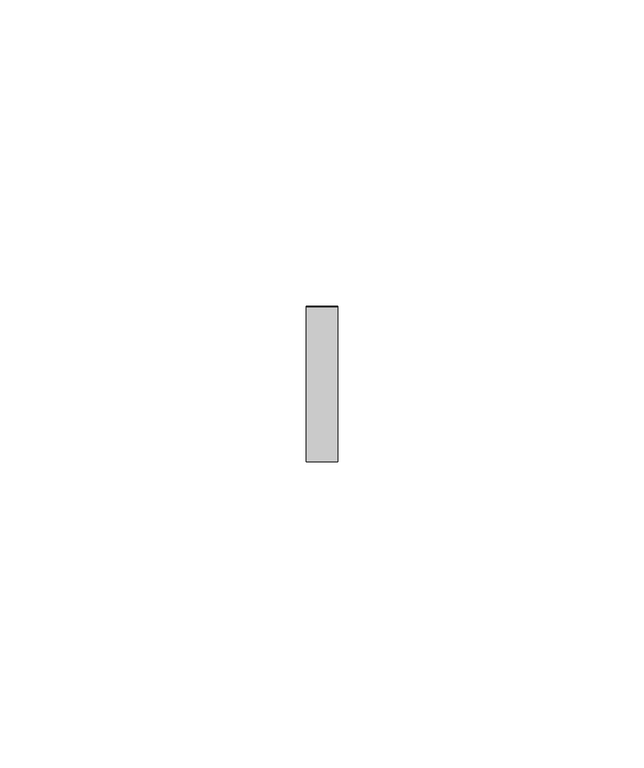
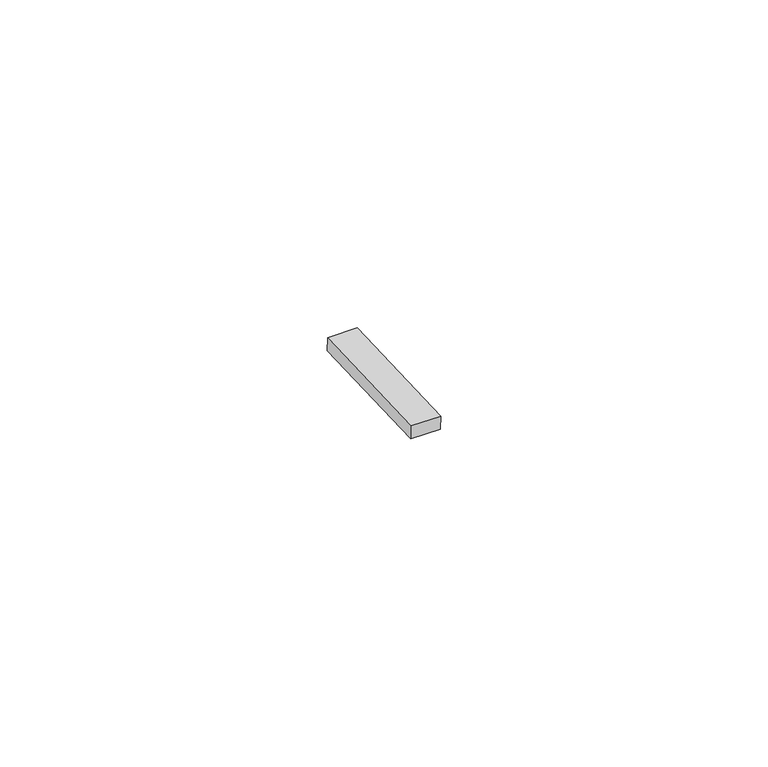
"""IFC4 building model written with IfcOpenShell, lengths in millimetres: proxy geometry, Inner panel:Inner panel:1:Inner panel:1 : Inner panel:Inner panel:300324:2:Inner panel:1:Inner panel:1 : Inner panel:Inner panel:300324:2 : Inner panel:Inner panel:1:Inner panel:1 : Inner panel:Inner panel:300324:300043:126 : Inner panel:Inner panel:1:Inner panel:1 : Inner panel:Inner panel:300324:2:Inner panel:1:Inner panel:1 : Inner panel:Inner panel:300324:2 : Inner panel:Inner panel:1:Inner panel:1 : Inner panel:Inner panel:300324:300043:308120."""

from ifc_helpers import new_model, si_unit, frame, origin, place, context, project, spatial, polyline, outline, extrude, source, transform, mapped, element, save


def generic_models_61f8d52a(model_context):
    return source(origin(), model_context, "Body", "SweptSolid", [
        extrude(outline(polyline([(0.0, -25.3999999), (0.0, 0.0), (5.2138089, 0.0), (5.2138089, -25.3999999), (0.0, -25.3999999)])), frame((593123.795117, -577413.7950993, 4016.01903), z_axis=(0.0, -0.041630544712223896, 0.9991330730923502), x_axis=(-1.0, 0.0, 0.0)), (0.0, 0.0, 1.0), 2.4763745),
    ])


if __name__ == "__main__":
    model = new_model("IFC4")
    model_context = context("Model", 3, world=origin())
    ifc_project = project(units=[si_unit("LENGTHUNIT", "METRE", prefix="MILLI")], contexts=[model_context])
    site = spatial("IfcSite", under=ifc_project)
    building = spatial("IfcBuilding", under=site)
    placement = place(None, origin())
    generic_models_shape = generic_models_61f8d52a(model_context)
    element("IfcBuildingElementProxy", 1, Name="Inner panel:Inner panel:1:Inner panel:1 : Inner panel:Inner panel:300324:2:Inner panel:1:Inner panel:1 : Inner panel:Inner panel:300324:2 : Inner panel:Inner panel:1:Inner panel:1 : Inner panel:Inner panel:300324:300043:126 : Inner panel:Inner panel:1:Inner panel:1 : Inner panel:Inner panel:300324:2:Inner panel:1:Inner panel:1 : Inner panel:Inner panel:300324:2 : Inner panel:Inner panel:1:Inner panel:1 : Inner panel:Inner panel:300324:300043:308120", ObjectType="Inner panel:Inner panel:1:Inner panel:1 : Inner panel:Inner panel:300324:2:Inner panel:1:Inner panel:1 : Inner panel:Inner panel:300324:2 : Inner panel:Inner panel:1:Inner panel:1 : Inner panel:Inner panel:300324:300043:126 : Inner panel:Inner panel:1:Inner panel:1 : Inner panel:Inner panel:300324:2:Inner panel:1:Inner panel:1 : Inner panel:Inner panel:300324:2 : Inner panel:Inner panel:1:Inner panel:1 : Inner panel:Inner panel:300324:300043:308120", at=placement, inside=building, context=model_context, shape_type="MappedRepresentation", body=[
        mapped(generic_models_shape, transform((0.0, 0.0, 0.0), x_axis=(1.0, 0.0, 0.0), y_axis=(0.0, 1.0, 0.0), z_axis=(0.0, 0.0, 1.0))),
    ])
    save(model, "model.ifc")

# Revit data of these elements
# Type "Inner panel:Inner panel:1:Inner panel:1 : Inner panel:Inner panel:300324:2:Inner panel:1:Inner panel:1 : Inner panel:Inner panel:300324:2 : Inner panel:Inner panel:1:Inner panel:1 : Inner panel:Inner panel:300324:300043:126 : Inner panel:Inner panel:1:Inner panel:1 : Inner panel:Inner panel:300324:2:Inner panel:1:Inner panel:1 : Inner panel:Inner panel:300324:2 : Inner panel:Inner panel:1:Inner panel:1 : Inner panel:Inner panel:300324:300043:308120"
#   NameOverride = "Inner panel:Inner panel:1:Inner panel:1 : Inner panel:Inner panel:300324:2:Inner panel:1:Inner panel:1 : Inner panel:Inner panel:300324:2 : Inner panel:Inner panel:1:Inner panel:1 : Inner panel:Inner panel:300324:300043:308120"
#   ObjectTypeOverride = "Inner panel:1:Inner panel:1 : Inner panel:Inner panel:300324:2 : Inner panel:Inner panel:1:Inner panel:1 : Inner panel:Inner panel:300324:300043"
#   Reference = "Inner panel"
#   Tag = "308120"
# Element 1 (IfcBuildingElementProxy, "Inner panel:Inner panel:1:Inner panel:1 : Inner panel:Inner panel:300324:2:Inner panel:1:Inner panel:1 : Inner panel:Inner panel:300324:2 : Inner panel:Inner panel:1:Inner panel:1 : Inner panel:Inner panel:300324:300043:126 : Inner panel:Inner panel:1:Inner panel:1 : Inner panel:Inner panel:300324:2:Inner panel:1:Inner panel:1 : Inner panel:Inner panel:300324:2 : Inner panel:Inner panel:1:Inner panel:1 : Inner panel:Inner panel:300324:300043:308120")
#   Materials on its faces: "AT CLIP - 1\" WIDE NON ABSORBENT, WEATHER-RESISTANT NEOPRENE/EPDM/SBR FOAM"
# Materials
#   "AT CLIP - 1\" WIDE NON ABSORBENT, WEATHER-RESISTANT NEOPRENE/EPDM/SBR FOAM": class "Generic", colour RGB 85 85 85, transparency 0, Cost = 0
